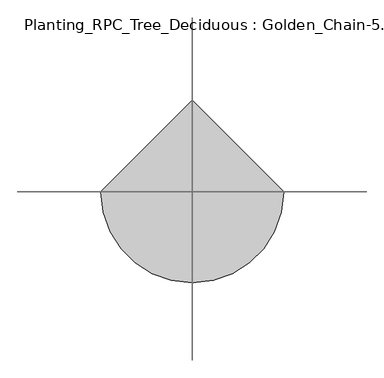
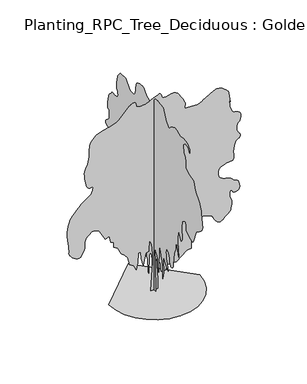
"""IFC4 building model written with IfcOpenShell, lengths in millimetres: geographic element geometry, Planting_RPC_Tree_Deciduous : Golden_Chain-5.5_Meters."""

from ifc_helpers import new_model, si_unit, origin, place, context, project, spatial, triangles, source, transform, mapped, element, save


def planting_rpc_tree_deciduous_golden_chain_5_5_meters_6778af60(model_context):
    return source(origin(), model_context, "Body", "Tessellation", [
        triangles([(-0.0021492, 84.2526153, 0.0017055), (-0.0021492, -79.7118042, 0.0017055), (-0.0021492, -55.1171299, 770.634066), (-0.0021492, -30.52271, 1205.1391577), (-0.0021492, -128.9011618, 1090.3648407), (-0.0021492, -161.6941456, 983.7870438), (-0.0021492, -161.6941456, 778.8331295), (-0.0021492, -202.6851937, 614.8669024), (-0.0021492, -227.2798771, 1410.0956154), (-0.0021492, -292.8648273, 1254.3285244), (-0.0021492, -391.2435245, 934.5977497), (-0.0021492, -407.6416878, 557.4810519), (-0.0021492, -448.6319547, 754.2384825), (-0.0021492, -424.0372713, 1123.1586239), (-0.0021492, -399.4426243, 1229.7338047), (-0.0021492, -563.4062716, 1024.7798904), (-0.0021492, -645.3893852, 910.00303), (-0.0021492, -571.6053351, 1164.1488544), (-0.0021492, -566.3701532, 1202.7023878), (-0.0021492, -561.3514189, 1240.6803749), (-0.0021492, -556.7629998, 1277.5125744), (-0.0021492, -552.8187638, 1312.6233673), (-0.0021492, -549.7351948, 1345.442585), (-0.0021492, -547.7261604, 1375.3895943), (-0.0021492, -547.0106518, 1401.8965519), (-0.0021492, -548.2048739, 1425.0576382), (-0.0021492, -551.550709, 1445.6369053), (-0.0021492, -556.6891308, 1464.0644142), (-0.0021492, -563.2636931, 1480.7706619), (-0.0021492, -570.9127539, 1496.1884708), (-0.0021492, -579.2773232, 1510.7457218), (-0.0021492, -588.000955, 1524.870005), (-0.0021492, -615.9185097, 1493.2475166), (-0.0021492, -642.6877333, 1461.6276443), (-0.0021492, -667.1627655, 1430.0051559), (-0.0021492, -688.1976734, 1398.3826675), (-0.0021492, -704.6416552, 1366.7627953), (-0.0021492, -715.3488504, 1335.1403069), (-0.0021492, -719.173399, 1303.5178185), (-0.0021492, -720.8463346, 1273.0922047), (-0.0021492, -725.5315138, 1244.8155876), (-0.0021492, -732.7248247, 1218.3340645), (-0.0021492, -741.9270973, 1193.2836313), (-0.0021492, -752.6342926, 1169.31024), (-0.0021492, -764.3472404, 1146.0549007), (-0.0021492, -776.5592857, 1123.1586239), (-0.0021492, -799.2416948, 1123.4208899), (-0.0021492, -820.9921841, 1125.2618385), (-0.0021492, -840.8787609, 1130.2576818), (-0.0021492, -857.9695055, 1139.9845591), (-0.0021492, -871.3298819, 1156.0210802), (-0.0021492, -880.0305862, 1179.9486168), (-0.0021492, -883.1370827, 1213.3382212), (-0.0021492, -884.8100183, 1255.5711811), (-0.0021492, -889.4951975, 1304.2589069), (-0.0021492, -896.6884357, 1358.3243568), (-0.0021492, -905.890781, 1416.6930325), (-0.0021492, -916.5979763, 1478.2854939), (-0.0021492, -928.3109241, 1542.0320389), (-0.0021492, -940.5255129, 1606.8530823), (-0.0021492, -1006.1104631, 1762.6177025), (-0.0021492, -1030.7051102, 2041.3581013), (-0.0021492, -1137.2829071, 1615.0495296), (-0.0021492, -1096.2900604, 2033.1590378), (-0.0021492, -1120.8847801, 2385.6835957), (-0.0021492, -1260.2563602, 2139.7368347), (-0.0021492, -1270.7241806, 2153.8611179), (-0.0021492, -1280.7616493, 2168.4183689), (-0.0021492, -1289.9410309, 2183.833707), (-0.0021492, -1297.8295029, 2200.5424255), (-0.0021492, -1303.9940975, 2218.9699345), (-0.0021492, -1308.0095501, 2239.5492016), (-0.0021492, -1309.4456543, 2262.7102879), (-0.0021492, -1307.6275967, 2290.0778034), (-0.0021492, -1302.9424175, 2322.033847), (-0.0021492, -1296.538448, 2357.1447853), (-0.0021492, -1289.5590775, 2393.9769848), (-0.0021492, -1283.1526371, 2431.0968121), (-0.0021492, -1278.467458, 2467.0683083), (-0.0021492, -1276.6518711, 2500.45784), (-0.0021492, -1277.8461296, 2532.7959824), (-0.0021492, -1281.1944717, 2566.4375336), (-0.0021492, -1286.3329662, 2601.1435547), (-0.0021492, -1292.9049488, 2636.6899315), (-0.0021492, -1300.5540459, 2672.8981865), (-0.0021492, -1308.9185062, 2709.5395546), (-0.0021492, -1317.642247, 2746.4096878), (-0.0021492, -1349.0965771, 2763.5973015), (-0.0021492, -1379.5477707, 2778.4931946), (-0.0021492, -1407.98993, 2788.7800667), (-0.0021492, -1433.4222439, 2792.1923584), (-0.0021492, -1454.8366344, 2786.4374771), (-0.0021492, -1471.2347614, 2769.1992851), (-0.0021492, -1481.6057854, 2738.2107697), (-0.0021492, -1484.4041611, 2701.900486), (-0.0021492, -1481.8935585, 2669.6135033), (-0.0021492, -1478.8100258, 2640.3309883), (-0.0021492, -1479.8871403, 2613.0602692), (-0.0021492, -1489.8532471, 2586.7825127), (-0.0021492, -1513.444685, 2560.5300453), (-0.0021492, -1555.3924152, 2533.2517685), (-0.0021492, -1606.8988644, 2505.0718025), (-0.0021492, -1655.253035, 2478.4681938), (-0.0021492, -1699.3015091, 2456.025087), (-0.0021492, -1737.903368, 2440.3219757), (-0.0021492, -1769.9076645, 2433.9411152), (-0.0021492, -1794.1662128, 2439.4615631), (-0.0021492, -1809.5357689, 2459.4676094), (-0.0021492, -1957.1037964, 2820.1761154), (-0.0021492, -2096.4727604, 2918.5648773), (-0.0021492, -2133.9033245, 2947.2108032), (-0.0021492, -2168.0337994, 2976.9770096), (-0.0021492, -2197.5760368, 3008.067263), (-0.0021492, -2221.2386913, 3040.5580124), (-0.0021492, -2237.731144, 3074.6530243), (-0.0021492, -2245.7620491, 3110.453746), (-0.0021492, -2244.0407879, 3148.1136566), (-0.0021492, -2235.2459759, 3194.9398682), (-0.0021492, -2223.869054, 3254.6760475), (-0.0021492, -2211.3438011, 3322.1530334), (-0.0021492, -2199.1063213, 3392.2013741), (-0.0021492, -2188.5901028, 3459.67836), (-0.0021492, -2181.2287788, 3519.4145393), (-0.0021492, -2178.4558376, 3566.2154617), (-0.0021492, -2170.3281361, 3608.6875786), (-0.0021492, -2147.5744377, 3658.060437), (-0.0021492, -2112.6315125, 3713.1367264), (-0.0021492, -2067.9338047, 3772.8217461), (-0.0021492, -2015.9257874, 3835.9446373), (-0.0021492, -1959.038998, 3901.3845383), (-0.0021492, -1899.7152935, 3967.9447197), (-0.0021492, -1842.3294067, 4197.4932083), (-0.0021492, -1629.1739582, 4246.6875893), (-0.0021492, -1457.0136818, 4328.652935), (-0.0021492, -1458.3505188, 4335.1970123), (-0.0021492, -1461.6963902, 4352.7409996), (-0.0021492, -1466.0480141, 4378.3565872), (-0.0021492, -1470.3970219, 4408.9631493), (-0.0021492, -1473.7428932, 4441.6065056), (-0.0021492, -1475.082201, 4473.2060303), (-0.0021492, -1473.409338, 4500.8334137), (-0.0021492, -1467.7438408, 4526.8565346), (-0.0021492, -1458.2079403, 4555.4515915), (-0.0021492, -1445.4433125, 4586.2107605), (-0.0021492, -1430.0993362, 4618.7015099), (-0.0021492, -1412.8176876, 4652.4654373), (-0.0021492, -1394.2474548, 4687.1205894), (-0.0021492, -1375.0306046, 4722.1829842), (-0.0021492, -1342.2368214, 4918.9352188), (-0.0021492, -1448.8146183, 5009.1250626), (-0.0021492, -1579.9871349, 4984.5277267), (-0.0021492, -1653.7685326, 4877.9400467), (-0.0021492, -1653.7685326, 4976.3288086), (-0.0021492, -1538.9942883, 5082.8914902), (-0.0021492, -1350.4358849, 5107.488826), (-0.0021492, -1202.8678574, 5074.692572), (-0.0021492, -1055.2998299, 5156.6829163), (-0.0021492, -948.7220329, 5164.8818344), (-0.0021492, -940.8819592, 5161.1390396), (-0.0021492, -920.1372952, 5151.1065125), (-0.0021492, -890.6409851, 5136.4911255), (-0.0021492, -856.5588358, 5118.9980072), (-0.0021492, -822.0437914, 5100.3334488), (-0.0021492, -791.2590425, 5082.280481), (-0.0021492, -768.3627657, 5066.4930725), (-0.0021492, -752.5400396, 5050.8591431), (-0.0021492, -739.1541561, 5033.7985565), (-0.0021492, -726.6289759, 5017.8844116), (-0.0021492, -713.3882143, 5005.6874817), (-0.0021492, -697.8532614, 4999.805864), (-0.0021492, -678.4453617, 5002.8359116), (-0.0021492, -653.5859053, 5017.2989822), (-0.0021492, -627.1527803, 5039.5790176), (-0.0021492, -603.7294281, 5064.0234558), (-0.0021492, -582.814135, 5090.2247635), (-0.0021492, -563.9078762, 5117.8777267), (-0.0021492, -546.5090472, 5146.6253906), (-0.0021492, -530.1108839, 5176.0602219), (-0.0021492, -514.2169049, 5205.8775879), (-0.0021492, -415.8382078, 5410.8290314), (-0.0021492, -169.8924643, 5451.8242035), (-0.0021492, -163.845268, 5451.6713058), (-0.0021492, -147.6161895, 5450.6783432), (-0.0021492, -124.0728773, 5447.9540909), (-0.0021492, -96.0842423, 5442.6323227), (-0.0021492, -66.5181736, 5433.8985535), (-0.0021492, -38.2425694, 5420.8359787), (-0.0021492, -14.1260625, 5402.6295319), (-0.0021492, 3.3458589, 5384.2457703), (-0.0021492, 15.2248406, 5370.0373352), (-0.0021492, 23.9488607, 5358.0950409), (-0.0021492, 31.9557643, 5346.6114395), (-0.0021492, 41.6836339, 5333.6761826), (-0.0021492, 55.5706269, 5317.4306625), (-0.0021492, 76.0543103, 5296.0418518), (-0.0021492, 97.13535, 5271.2916183), (-0.0021492, 113.1971331, 5247.5349289), (-0.0021492, 127.2514169, 5226.7827072), (-0.0021492, 142.3091915, 5211.0464584), (-0.0021492, 161.3827366, 5202.3638489), (-0.0021492, 187.483033, 5202.6946426), (-0.0021492, 223.6221062, 5214.076506), (-0.0021492, 264.351397, 5233.7851868), (-0.0021492, 302.4974698, 5257.3889786), (-0.0021492, 338.4919115, 5284.2012955), (-0.0021492, 372.7676173, 5313.5855484), (-0.0021492, 405.7523409, 5344.9307281), (-0.0021492, 437.8763975, 5377.549086), (-0.0021492, 469.5675954, 5410.8290314), (-0.0021492, 492.466452, 5419.4860611), (-0.0021492, 515.7217913, 5427.3286057), (-0.0021492, 539.6951463, 5433.618338), (-0.0021492, 564.7456158, 5437.5396103), (-0.0021492, 591.2271026, 5438.3035172), (-0.0021492, 619.503756, 5435.1205719), (-0.0021492, 649.9294424, 5427.2268677), (-0.0021492, 681.4067362, 5417.9076691), (-0.0021492, 712.0259428, 5409.8610672), (-0.0021492, 740.9213448, 5401.4075134), (-0.0021492, 767.2373257, 5390.7895569), (-0.0021492, 790.1107115, 5376.3009064), (-0.0021492, 808.6833424, 5356.2364334), (-0.0021492, 822.0921896, 5328.8381058), (-0.0021492, 831.6764156, 5297.4679276), (-0.0021492, 839.5393805, 5266.5047012), (-0.0021492, 845.9687845, 5235.9240097), (-0.0021492, 851.2523283, 5205.5973724), (-0.0021492, 855.672698, 5175.5253708), (-0.0021492, 859.522681, 5145.5556885), (-0.0021492, 863.0824202, 5115.6877441), (-0.0021492, 868.5086151, 5085.9976959), (-0.0021492, 874.8667299, 5057.4029297), (-0.0021492, 883.0886845, 5030.9469864), (-0.0021492, 894.1065439, 5007.6989868), (-0.0021492, 908.8546263, 4988.7803741), (-0.0021492, 928.2625259, 4975.2085281), (-0.0021492, 953.2646336, 4968.1298904), (-0.0021492, 983.5706326, 4964.7940475), (-0.0021492, 1017.0340696, 4962.6296448), (-0.0021492, 1051.7859455, 4962.7313828), (-0.0021492, 1085.9648186, 4966.2962814), (-0.0021492, 1117.7069944, 4974.4446213), (-0.0021492, 1145.1458719, 4988.347261), (-0.0021492, 1166.4176113, 5009.1250626), (-0.0021492, 1187.9516893, 5037.6180908), (-0.0021492, 1215.2250246, 5071.5857849), (-0.0021492, 1244.9327316, 5107.4120865), (-0.0021492, 1273.7822788, 5141.5326782), (-0.0021492, 1298.4736496, 5170.3309204), (-0.0021492, 1315.7070454, 5190.2430771), (-0.0021492, 1322.1822315, 5197.6786697), (-0.0021492, 1576.328056, 5181.2802521), (-0.0021492, 1674.7067894, 5058.2941544), (-0.0021492, 1679.9878624, 5049.3057495), (-0.0021492, 1685.3426228, 5039.1203247), (-0.0021492, 1690.840107, 5026.4652832), (-0.0021492, 1696.5540024, 5010.1691849), (-0.0021492, 1702.550584, 4988.9838501), (-0.0021492, 1708.9086262, 4961.7134216), (-0.0021492, 1715.69702, 4927.1347183), (-0.0021492, 1722.2461842, 4888.9655365), (-0.0021492, 1727.9344997, 4851.6622902), (-0.0021492, 1732.907452, 4815.0465019), (-0.0021492, 1737.304858, 4779.0417229), (-0.0021492, 1741.2720577, 4743.4444771), (-0.0021492, 1744.9539551, 4708.1530266), (-0.0021492, 1748.4908031, 4672.9886032), (-0.0021492, 1731.0893944, 4648.3403984), (-0.0021492, 1714.6937382, 4623.4122688), (-0.0021492, 1700.3046455, 4597.9237083), (-0.0021492, 1688.927869, 4571.5442139), (-0.0021492, 1681.5665451, 4544.0441483), (-0.0021492, 1679.2239555, 4515.0927177), (-0.0021492, 1682.9058529, 4484.4352867), (-0.0021492, 1691.9172215, 4457.546521), (-0.0021492, 1704.798848, 4438.9584114), (-0.0021492, 1721.4109154, 4426.9908279), (-0.0021492, 1741.6082291, 4419.8866104), (-0.0021492, 1765.2454491, 4415.940049), (-0.0021492, 1792.1827583, 4413.4445618), (-0.0021492, 1822.2748169, 4410.6435699), (-0.0021492, 1851.5776794, 4410.5162521), (-0.0021492, 1877.0099934, 4414.7177399), (-0.0021492, 1899.7152935, 4419.453788), (-0.0021492, 1920.8445271, 4421.0580505), (-0.0021492, 1941.543409, 4415.7871513), (-0.0021492, 1962.9576542, 4399.8982956), (-0.0021492, 1986.2385006, 4369.6483978), (-0.0021492, 2009.8529022, 4339.016256), (-0.0021492, 2031.6033188, 4320.2755394), (-0.0021492, 2051.6324741, 4307.2641243), (-0.0021492, 2070.0854176, 4293.8451759), (-0.0021492, 2087.1024021, 4273.8057014), (-0.0021492, 2102.8308025, 4241.0094475), (-0.0021492, 2117.4110172, 4189.2939995), (-0.0021492, 2130.4606567, 4132.1297562), (-0.0021492, 2141.5040234, 4085.4561516), (-0.0021492, 2150.5382103, 4046.6759605), (-0.0021492, 2157.565979, 4013.1922485), (-0.0021492, 2162.5848587, 3982.4330795), (-0.0021492, 2165.5945587, 3951.8009377), (-0.0021492, 2166.6003113, 3918.7500481), (-0.0021492, 2163.9699486, 3888.1437767), (-0.0021492, 2156.6086246, 3865.7361328), (-0.0021492, 2145.3030647, 3850.1274925), (-0.0021492, 2130.8426102, 3839.9676476), (-0.0021492, 2114.0167477, 3833.9075523), (-0.0021492, 2095.6120571, 3830.5464203), (-0.0021492, 2076.4181705, 3828.5602043), (-0.0021492, 2076.4181705, 3615.4098427), (-0.0021492, 2076.5861835, 3611.7687859), (-0.0021492, 2077.7574783, 3607.2362137), (-0.0021492, 2080.9351913, 3600.9979317), (-0.0021492, 2087.1278366, 3592.1877136), (-0.0021492, 2097.3334637, 3579.9143349), (-0.0021492, 2112.5576797, 3563.3636009), (-0.0021492, 2133.8065281, 3541.6437057), (-0.0021492, 2158.6890209, 3518.8288193), (-0.0021492, 2183.2835953, 3498.7640556), (-0.0021492, 2206.2996323, 3480.0997879), (-0.0021492, 2226.4484024, 3461.6134163), (-0.0021492, 2242.4391415, 3441.9561859), (-0.0021492, 2252.9807945, 3419.8796265), (-0.0021492, 2256.7799812, 3394.0602722), (-0.0021492, 2250.3276134, 3369.7687317), (-0.0021492, 2232.2566235, 3352.3773514), (-0.0021492, 2204.5070091, 3340.7152725), (-0.0021492, 2169.0142628, 3333.6366348), (-0.0021492, 2127.7106792, 3329.995578), (-0.0021492, 2082.5368378, 3328.6715309), (-0.0021492, 2035.4277946, 3328.4677643), (-0.0021492, 2021.5658501, 3329.995578), (-0.0021492, 2008.8496204, 3330.1737648), (-0.0021492, 1998.4275822, 3327.6274086), (-0.0021492, 1991.4508278, 3320.9815933), (-0.0021492, 1989.05984, 3308.886692), (-0.0021492, 1992.405566, 3289.9677887), (-0.0021492, 2002.6366276, 3262.9005455), (-0.0021492, 2020.3945553, 3234.9676575), (-0.0021492, 2044.3195484, 3213.2224731), (-0.0021492, 2072.5477673, 3195.7802238), (-0.0021492, 2103.212756, 3180.7570129), (-0.0021492, 2134.4508202, 3166.3195221), (-0.0021492, 2164.4003002, 3150.6088531), (-0.0021492, 2191.195031, 3131.7155296), (-0.0021492, 2214.6667088, 3115.4700096), (-0.0021492, 2235.4113728, 3106.0996513), (-0.0021492, 2252.7159851, 3099.4538361), (-0.0021492, 2265.8625664, 3091.381945), (-0.0021492, 2274.1329918, 3077.7083611), (-0.0021492, 2276.8091366, 3054.2824654), (-0.0021492, 2273.1754921, 3016.9539299), (-0.0021492, 2263.7593517, 2975.5765137), (-0.0021492, 2250.0398403, 2941.939904), (-0.0021492, 2232.735228, 2914.7709229), (-0.0021492, 2212.5634941, 2892.7455231), (-0.0021492, 2190.2375313, 2874.6158157), (-0.0021492, 2166.4806965, 2859.0580444), (-0.0021492, 2142.0055916, 2844.7731606), (-0.0021492, 2133.3761765, 2827.1783043), (-0.0021492, 2125.6812973, 2809.2779434), (-0.0021492, 2119.8477871, 2790.7918625), (-0.0021492, 2116.8125072, 2771.4654259), (-0.0021492, 2117.5051975, 2750.9675491), (-0.0021492, 2122.8599579, 2729.044178), (-0.0021492, 2133.8065281, 2705.4145157), (-0.0021492, 2153.6931049, 2682.9815826), (-0.0021492, 2182.4714355, 2663.4005104), (-0.0021492, 2215.980582, 2644.532476), (-0.0021492, 2250.062804, 2624.2386566), (-0.0021492, 2280.5623959, 2600.3543587), (-0.0021492, 2303.3160942, 2570.7407593), (-0.0021492, 2314.1683388, 2533.2517685), (-0.0021492, 2316.6306885, 2491.7827881), (-0.0021492, 2316.7960854, 2450.4562408), (-0.0021492, 2314.3822792, 2407.4085777), (-0.0021492, 2309.1012062, 2360.7782845), (-0.0021492, 2300.6627678, 2308.6964344), (-0.0021492, 2288.7842777, 2249.3015133), (-0.0021492, 2273.1754921, 2180.7272106), (-0.0021492, 2256.9479942, 2122.3126076), (-0.0021492, 2242.7269146, 2087.8459614), (-0.0021492, 2229.5091167, 2067.1470795), (-0.0021492, 2216.2913189, 2050.0334438), (-0.0021492, 2202.0702393, 2026.3248619), (-0.0021492, 2185.8401253, 1985.8335835), (-0.0021492, 2166.6003113, 1918.3847935), (-0.0021492, 2149.5808559, 1842.5203835), (-0.0021492, 2138.8736607, 1783.2936207), (-0.0021492, 2131.7517117, 1740.2713921), (-0.0021492, 2125.4903206, 1713.0234913), (-0.0021492, 2117.362619, 1701.1195667), (-0.0021492, 2104.6463894, 1704.1317375), (-0.0021492, 2084.617234, 1721.6273266), (-0.0021492, 2060.5012642, 1758.0775726), (-0.0021492, 2037.2458523, 1813.4570412), (-0.0021492, 2014.7060944, 1880.5977104), (-0.0021492, 1992.7391212, 1952.324437), (-0.0021492, 1971.2051159, 2021.4716698), (-0.0021492, 1949.9562675, 2080.8664455), (-0.0021492, 1928.8526138, 2123.3387077), (-0.0021492, 1903.2291779, 2154.4824463), (-0.0021492, 1869.4322582, 2184.7680977), (-0.0021492, 1828.8238358, 2214.3331535), (-0.0021492, 1782.7664726, 2243.3252792), (-0.0021492, 1732.6196789, 2271.8870533), (-0.0021492, 1679.7509583, 2300.1636703), (-0.0021492, 1625.51735, 2328.2952381), (-0.0021492, 1580.1042789, 2357.6693172), (-0.0021492, 1536.2697453, 2384.1049129), (-0.0021492, 1495.5901062, 2404.6612164), (-0.0021492, 1459.6414284, 2416.3971279), (-0.0021492, 1430.0025398, 2416.3715481), (-0.0021492, 1408.2521233, 2401.6489002), (-0.0021492, 1395.9662453, 2369.2854687), (-0.0021492, 1387.7442181, 2327.3633183), (-0.0021492, 1377.3731941, 2285.8713741), (-0.0021492, 1365.2069309, 2244.7359489), (-0.0021492, 1351.6071796, 2203.8882969), (-0.0021492, 1336.9303139, 2163.2544399), (-0.0021492, 1321.5379395, 2122.7657776), (-0.0021492, 1305.7865753, 2082.3484772), (-0.0021492, 1125.4248373, 1926.583857), (-0.0021492, 1107.9775738, 1907.1276318), (-0.0021492, 1091.2458916, 1886.8820652), (-0.0021492, 1075.9502409, 1865.0602867), (-0.0021492, 1062.8037323, 1840.8729549), (-0.0021492, 1052.5268887, 1813.5282578), (-0.0021492, 1045.8352186, 1782.2419407), (-0.0021492, 1043.4442308, 1746.2220463), (-0.0021492, 1042.7261787, 1711.1595062), (-0.0021492, 1040.7196878, 1682.5468632), (-0.0021492, 1037.6361551, 1659.3168858), (-0.0021492, 1033.6919191, 1640.3851925), (-0.0021492, 1029.1035364, 1624.6822266), (-0.0021492, 1024.0847294, 1611.1308735), (-0.0021492, 1018.8495838, 1598.6540188), (-0.0021492, 871.2814837, 1500.2752853), (-0.0021492, 854.8859001, 1328.1125381), (-0.0021492, 731.9125196, 1270.7241806), (-0.0021492, 699.1188091, 1057.5711302), (-0.0021492, 567.9463288, 1024.7798904), (-0.0021492, 579.9928319, 1019.3537682), (-0.0021492, 590.5345213, 1012.9956533), (-0.0021492, 598.0638946, 1004.7736261), (-0.0021492, 601.0736309, 993.7558393), (-0.0021492, 598.0638946, 979.0076843), (-0.0021492, 587.5222415, 959.5997847), (-0.0021492, 567.9463288, 934.5977497), (-0.0021492, 544.3090362, 908.8801334), (-0.0021492, 522.3905339, 887.4631994), (-0.0021492, 501.9081359, 869.6340551), (-0.0021492, 482.5715618, 854.6720324), (-0.0021492, 464.0956183, 841.8616224), (-0.0021492, 446.192605, 830.4822298), (-0.0021492, 428.5773285, 819.8234327), (-0.0021492, 416.3169213, 852.4974558), (-0.0021492, 404.2703819, 880.9396151), (-0.0021492, 392.6541942, 900.9203722), (-0.0021492, 381.6821895, 908.2104795), (-0.0021492, 371.5733952, 898.5777826), (-0.0021492, 362.5365921, 867.7931065), (-0.0021492, 354.7933147, 811.6243692), (-0.0021492, 347.289376, 757.5588467), (-0.0021492, 338.9222268, 728.4470335), (-0.0021492, 329.8396053, 713.1030573), (-0.0021492, 320.1840537, 700.3409729), (-0.0021492, 310.0981504, 678.9725098), (-0.0021492, 299.7245467, 637.8141209), (-0.0021492, 289.2083463, 565.677572), (-0.0021492, 280.1002358, 485.3215393), (-0.0021492, 273.5766333, 424.7553234), (-0.0021492, 269.2021002, 380.6814875), (-0.0021492, 266.5488464, 349.8000149), (-0.0021492, 265.1865749, 328.815976), (-0.0021492, 264.6849704, 314.426847), (-0.0021492, 264.613663, 303.3351912), (-0.0021492, 240.0187434, 811.6243692), (-0.0021492, 227.6618124, 844.6574547), (-0.0021492, 214.9461096, 875.6102165), (-0.0021492, 201.5133903, 902.4023312), (-0.0021492, 187.005355, 922.9585619), (-0.0021492, 171.062996, 935.1961143), (-0.0021492, 153.328032, 937.037063), (-0.0021492, 133.4419729, 926.401157), (-0.0021492, 115.707018, 904.291678), (-0.0021492, 103.9950694, 874.0085701), (-0.0021492, 97.3026454, 836.9141773), (-0.0021492, 94.6257194, 794.3680824), (-0.0021492, 94.9603011, 747.7377892), (-0.0021492, 97.3026454, 698.3803368), (-0.0021492, 100.6487348, 647.6606855), (-0.0021492, 84.2526153, 237.7499866), (88.4435659, 0.0002505, 0.0), (-86.3932913, 0.0002505, 0.0), (-44.7656723, 0.0002025, 807.5807934), (-36.4400473, 0.0001919, 1032.3704155), (-69.7422955, 0.0001759, 1307.1158546), (-128.0216733, 0.0001652, 1448.6490761), (-144.6726646, 0.0001865, 1140.6032713), (-227.9278935, 0.0001865, 1115.6266708), (-294.532658, 0.0002025, 799.2544121), (-352.8122947, 0.0001919, 999.0699772), (-361.138676, 0.0001812, 1182.2301636), (-427.7421324, 0.0001812, 1182.2301636), (-444.3923879, 0.0001972, 915.8137218), (-486.0217873, 0.0002079, 732.6509193), (-552.6252437, 0.0002025, 874.1842861), (-660.8581358, 0.0001972, 940.7903223), (-702.4849554, 0.0001812, 1157.2534904), (-785.7412107, 0.0001759, 1257.1625084), (-877.3238474, 0.0001759, 1332.0923824), (-977.2303219, 0.0001599, 1523.5789501), (-1085.4632504, 0.0001599, 1581.8586777), (-1085.4632504, 0.0001492, 1723.3945152), (-1160.3931244, 0.0001492, 1748.3711884), (-1202.019944, 0.0001386, 1939.857756), (-1318.5792538, 0.0001386, 1889.9044098), (-1468.4390018, 0.0001226, 2172.9736141), (-1502.3250149, 0.0001226, 2194.0442757), (-1536.1347244, 0.0001226, 2213.0727654), (-1569.8018555, 0.0001173, 2228.0246143), (-1603.2501045, 0.0001173, 2236.8602669), (-1636.4053482, 0.0001173, 2237.5401672), (-1669.1991314, 0.0001173, 2228.0246143), (-1701.5548599, 0.0001226, 2206.2766685), (-1733.4726791, 0.0001226, 2179.018594), (-1764.2269066, 0.0001226, 2153.3621658), (-1792.651189, 0.0001279, 2127.850787), (-1817.579464, 0.0001279, 2101.0306217), (-1837.8479942, 0.0001279, 2071.4426022), (-1852.2879559, 0.0001332, 2037.6304218), (-1859.7409893, 0.0001332, 1998.1373383), (-1862.0709343, 0.0001386, 1954.9318359), (-1863.0894768, 0.0001386, 1911.4359444), (-1864.5459286, 0.0001439, 1868.3754913), (-1868.1871307, 0.0001439, 1826.4812462), (-1875.759779, 0.0001439, 1786.4790367), (-1889.0133305, 0.0001492, 1749.0993416), (-1909.6943356, 0.0001492, 1715.0681339), (-1930.6655846, 0.0001546, 1683.7079842), (-1945.9586918, 0.0001546, 1654.8226833), (-1959.0644325, 0.0001546, 1629.87159), (-1973.4840466, 0.0001546, 1610.3057785), (-1992.7085999, 0.0001599, 1597.5870781), (-2020.2341, 0.0001599, 1593.1693245), (-2059.5539383, 0.0001599, 1598.5088242), (-2106.0849644, 0.0001546, 1614.4818317), (-2151.4523987, 0.0001546, 1639.6289886), (-2193.4662586, 0.0001546, 1671.9108845), (-2229.9496422, 0.0001492, 1709.2905796), (-2258.7125668, 0.0001492, 1749.7308437), (-2277.5730434, 0.0001439, 1791.1870342), (-2284.3435604, 0.0001439, 1831.6274437), (-2284.0049183, 0.0001439, 1867.2347179), (-2283.6662762, 0.0001386, 1899.34613), (-2284.3435604, 0.0001386, 1933.6447632), (-2287.0630165, 0.0001332, 1975.8062885), (-2292.8405708, 0.0001332, 2031.5116093), (-2302.6947659, 0.0001279, 2106.4440994), (-2317.6466148, 0.0001226, 2206.2766685), (-2328.3767738, 0.0001119, 2318.4664776), (-2327.0169731, 0.0001066, 2424.8304794), (-2316.773267, 0.0001013, 2522.6006744), (-2300.8512737, 9.59e-05, 2609.0116791), (-2282.4516701, 9.06e-05, 2681.301162), (-2264.780365, 9.06e-05, 2736.6829559), (-2251.0431221, 8.53e-05, 2772.4075195), (-2228.7604706, 8.53e-05, 2807.0370918), (-2187.9815643, 7.99e-05, 2856.639006), (-2135.6984184, 7.99e-05, 2914.8473717), (-2078.9007225, 7.46e-05, 2975.2454292), (-2024.5780209, 7.46e-05, 3031.4167099), (-1979.7200031, 6.93e-05, 3076.9444542), (-1951.3211552, 6.93e-05, 3105.4374825), (-1924.2819626, 6.4e-05, 3127.0812195), (-1882.823156, 6.4e-05, 3155.2940323), (-1832.9183533, 6.4e-05, 3188.4469505), (-1780.5385563, 5.86e-05, 3224.9607101), (-1731.6521507, 5.86e-05, 3263.2060501), (-1692.2328999, 5.33e-05, 3301.6042877), (-1668.2519508, 5.33e-05, 3338.5511604), (-1656.1646072, 5.33e-05, 3371.3218346), (-1648.0088551, 4.8e-05, 3398.84748), (-1643.1300831, 4.8e-05, 3421.9931602), (-1640.8716454, 4.8e-05, 3441.6759705), (-1640.5812561, 4.8e-05, 3458.7106865), (-1641.5997986, 4.8e-05, 3473.988533), (-1643.2752777, 4.26e-05, 3488.4260239), (-1673.4947994, 4.26e-05, 3483.4862091), (-1703.0597099, 4.26e-05, 3481.1180397), (-1731.3135086, 4.26e-05, 3483.8172935), (-1757.6014389, 4.26e-05, 3494.1806145), (-1781.2667095, 4.26e-05, 3514.7546494), (-1801.6574707, 4.26e-05, 3548.0601746), (-1818.1141697, 3.73e-05, 3596.6435463), (-1832.6281094, 3.2e-05, 3658.2386238), (-1846.5614159, 3.2e-05, 3726.3519081), (-1858.3075012, 2.66e-05, 3797.4190819), (-1866.2698059, 2.13e-05, 3867.7223488), (-1868.8440674, 1.6e-05, 3933.671521), (-1864.4261684, 1.6e-05, 3991.625251), (-1851.414608, 1.07e-05, 4037.8913223), (-1831.8514126, 1.07e-05, 4080.6180748), (-1810.1034668, 5.3e-06, 4129.8889046), (-1788.0628063, 5.3e-06, 4185.1436714), (-1767.626263, 0.0, 4245.7710754), (-1750.6831112, -5.3e-06, 4311.2106857), (-1739.1280025, -1.07e-05, 4380.8773636), (-1734.8579144, -1.07e-05, 4454.1853889), (-1735.4894165, -1.6e-05, 4523.877356), (-1735.8280586, -2.13e-05, 4584.5303398), (-1733.5466572, -2.13e-05, 4638.3334511), (-1726.3125057, -2.66e-05, 4687.5025429), (-1711.7987114, -3.2e-05, 4734.1761475), (-1687.6699516, -3.2e-05, 4780.5442474), (-1651.601659, -3.73e-05, 4828.8218239), (-1604.6581581, -3.73e-05, 4875.2407928), (-1551.3056007, -4.26e-05, 4914.6575729), (-1494.3144573, -4.26e-05, 4947.2247711), (-1436.4472046, -4.26e-05, 4973.1202835), (-1380.4746037, -4.26e-05, 4992.421431), (-1329.161602, -4.8e-05, 5005.3566879), (-1285.2761993, -4.8e-05, 5012.0022125), (-1238.819006, -4.8e-05, 5019.8197586), (-1181.7285227, -4.8e-05, 5034.7665207), (-1119.6854347, -4.8e-05, 5054.8059952), (-1058.3731888, -4.8e-05, 5077.9260956), (-1003.4673832, -5.33e-05, 5102.03974), (-960.651392, -5.33e-05, 5125.1598404), (-935.6009588, -5.33e-05, 5145.1993149), (-669.1845171, -6.93e-05, 5428.27099), (-646.0030106, -6.93e-05, 5444.1601364), (-622.8954094, -7.46e-05, 5458.928421), (-599.9328938, -7.46e-05, 5471.5328842), (-577.1893693, -7.46e-05, 5480.8520828), (-554.7386684, -7.46e-05, 5485.7918976), (-532.6495734, -7.46e-05, 5485.2826263), (-510.9983877, -7.46e-05, 5478.2295685), (-495.8275477, -7.46e-05, 5462.4933197), (-489.5407585, -6.93e-05, 5439.0418442), (-486.7500132, -6.93e-05, 5411.3888809), (-482.064834, -6.93e-05, 5382.9725922), (-470.0972506, -6.93e-05, 5357.3567139), (-445.4618357, -6.4e-05, 5337.9794083), (-402.7655319, -6.4e-05, 5328.3544144), (-352.1553217, -6.4e-05, 5326.9794983), (-306.7905035, -6.4e-05, 5329.5258545), (-265.7951497, -6.4e-05, 5335.3568939), (-228.2925333, -6.4e-05, 5343.8104477), (-193.4123404, -6.4e-05, 5354.2249283), (-160.2801876, -6.93e-05, 5365.9375854), (-128.0216733, -6.93e-05, 5378.3124115), (-76.4902348, -6.93e-05, 5408.3588333), (-26.1968067, -6.93e-05, 5436.7501236), (21.6206779, -7.46e-05, 5461.7805725), (65.7244948, -7.46e-05, 5481.7688873), (104.8766017, -7.46e-05, 5495.0605179), (137.8389157, -7.46e-05, 5500.0003326), (163.3739486, -7.46e-05, 5494.8820404), (179.7578323, -7.46e-05, 5482.2525787), (188.4231282, -7.46e-05, 5466.2872742), (192.8648993, -7.46e-05, 5447.6994553), (196.5786624, -6.93e-05, 5427.2012878), (203.0594986, -6.93e-05, 5405.5578415), (215.8026888, -6.93e-05, 5383.4562836), (238.3035501, -6.93e-05, 5361.6599396), (275.7078804, -6.4e-05, 5352.0093658), (327.5301169, -6.93e-05, 5359.8263306), (388.8194718, -6.93e-05, 5376.0974304), (454.6234131, -6.93e-05, 5391.7569397), (519.9893723, -6.93e-05, 5397.8426147), (579.9673974, -6.93e-05, 5385.2643127), (629.6048836, -6.4e-05, 5345.0068863), (669.510442, -6.4e-05, 5289.625383), (704.1731518, -5.86e-05, 5237.2989258), (734.4638901, -5.86e-05, 5187.5188248), (761.2611643, -5.33e-05, 5139.7758087), (785.4382496, -5.33e-05, 5093.5606064), (807.8660231, -4.8e-05, 5048.3633652), (829.420376, -4.8e-05, 5003.6759766), (821.0939947, -3.73e-05, 4853.8011131), (1104.163199, -3.73e-05, 4837.1483505), (1130.912075, -3.73e-05, 4839.0834068), (1157.5870457, -3.73e-05, 4841.7826607), (1184.116967, -3.73e-05, 4846.1111755), (1210.4303318, -3.73e-05, 4852.8334396), (1236.4509819, -3.73e-05, 4862.7639381), (1262.10741, -3.73e-05, 4876.6921577), (1287.3259289, -3.73e-05, 4895.433165), (1317.642247, -4.26e-05, 4918.5532654), (1357.5732399, -4.26e-05, 4944.7039948), (1405.5097034, -4.26e-05, 4973.4260788), (1459.8579849, -4.8e-05, 5004.1852478), (1519.010915, -4.8e-05, 5036.4722305), (1581.3671379, -4.8e-05, 5069.7527573), (1645.3250072, -5.33e-05, 5103.5675537), (1684.4540142, -5.33e-05, 5099.8497574), (1722.8521065, -5.33e-05, 5095.2663162), (1759.7963631, -5.33e-05, 5088.9515854), (1794.5558693, -4.8e-05, 5079.9887604), (1826.3998558, -4.8e-05, 5067.5371948), (1854.6051109, -4.8e-05, 5050.7062454), (1878.4410107, -4.8e-05, 5028.6552658), (1900.2143909, -4.8e-05, 5007.1897156), (1922.1329659, -4.26e-05, 4990.5372437), (1943.3232422, -4.26e-05, 4975.3358459), (1962.9118721, -4.26e-05, 4958.2502609), (1980.023037, -4.26e-05, 4935.9190659), (1993.7857143, -3.73e-05, 4905.0069992), (2003.3267017, -3.73e-05, 4862.1273491), (2036.62714, -2.13e-05, 4620.6877258), (2031.3358932, -2.66e-05, 4643.2223969), (2026.4088684, -2.66e-05, 4661.7340576), (2022.2099968, -2.66e-05, 4672.2502762), (2019.1035004, -2.66e-05, 4670.7477516), (2017.450985, -2.66e-05, 4653.2293442), (2017.6216141, -2.13e-05, 4615.6714622), (2019.9769936, -2.13e-05, 4554.0766754), (2029.0544918, -1.6e-05, 4483.8242775), (2046.7257969, -1.07e-05, 4423.1715843), (2069.3470905, -5.3e-06, 4372.5511276), (2093.2796413, -5.3e-06, 4332.4213097), (2114.8825378, -5.3e-06, 4303.2408234), (2130.5141418, -5.3e-06, 4285.3913315), (2136.5336872, 0.0, 4279.3565254), (2147.5539448, 0.0, 4280.1460121), (2175.7593452, 0.0, 4279.6367409), (2213.8671936, 0.0, 4273.4493279), (2254.5977016, 0.0, 4257.2038078), (2290.6659943, 0.0, 4226.5463768), (2314.794754, 5.3e-06, 4177.0973602), (2319.6963444, 1.07e-05, 4104.5023727), (2308.0216209, 1.07e-05, 4035.0650414), (2289.5024025, 1.6e-05, 3991.3959045), (2267.4871765, 1.6e-05, 3963.6159142), (2245.3241398, 1.6e-05, 3941.7939903), (2226.3694828, 2.13e-05, 3916.0255051), (2213.96399, 2.13e-05, 3876.4308289), (2211.466032, 2.66e-05, 3813.104171), (2219.5963497, 2.66e-05, 3747.2826073), (2234.7188278, 3.2e-05, 3702.4167412), (2253.6250866, 3.2e-05, 3671.9886566), (2273.1169201, 3.73e-05, 3649.4284058), (2289.9862392, 3.73e-05, 3628.141333), (2301.0320766, 3.73e-05, 3601.6598099), (2303.0461979, 4.26e-05, 3563.3380211), (2294.2843781, 4.26e-05, 3529.0395332), (2276.7837021, 4.26e-05, 3512.233873), (2253.0190189, 4.26e-05, 3502.8382256), (2225.4707005, 4.26e-05, 3490.8194824), (2196.6083633, 4.8e-05, 3466.1204086), (2168.9148502, 4.8e-05, 3418.7340569), (2144.8600685, 5.33e-05, 3338.5511604), (2129.882785, 5.86e-05, 3243.8796135), (2124.958231, 6.4e-05, 3160.284716), (2125.8545425, 6.93e-05, 3088.6321129), (2128.3549713, 7.46e-05, 3029.812738), (2128.2327404, 7.46e-05, 2984.6666565), (2121.2660145, 7.46e-05, 2954.0856743), (2103.2331036, 7.99e-05, 2938.9351456), (2080.3674934, 7.99e-05, 2933.5625084), (2059.979203, 7.99e-05, 2930.6853584), (2039.4433926, 7.99e-05, 2928.6482735), (2016.1421986, 7.99e-05, 2925.9237305), (1987.4504906, 7.99e-05, 2920.8565979), (1950.7506958, 7.99e-05, 2911.8426132), (1903.4176838, 7.99e-05, 2897.3033844), (1853.5127357, 7.99e-05, 2880.1413506), (1811.035532, 7.99e-05, 2862.9793167), (1776.2784966, 8.53e-05, 2843.7801979), (1749.5296932, 8.53e-05, 2820.5069092), (1731.0818367, 8.53e-05, 2791.0973671), (1721.2276417, 9.06e-05, 2753.5647743), (1720.2574974, 9.06e-05, 2705.8217583), (1723.631274, 9.59e-05, 2658.5115646), (1727.8785439, 9.59e-05, 2621.9722252), (1734.8910519, 9.59e-05, 2593.7338326), (1746.5683914, 0.0001013, 2571.3520592), (1764.7947498, 0.0001013, 2552.2802582), (1791.4723366, 0.0001013, 2534.1046234), (1828.4878098, 0.0001013, 2514.3224007), (1873.0047146, 0.0001013, 2496.0453186), (1919.5611752, 0.0001066, 2482.2824959), (1966.1151649, 0.0001066, 2470.414325), (2010.6320698, 0.0001066, 2457.815094), (2051.0697178, 0.0001066, 2441.8678116), (2085.3913147, 0.0001066, 2419.9517075), (2111.5570141, 0.0001119, 2389.4394711), (2135.660194, 0.0001119, 2361.79174), (2163.6949654, 0.0001119, 2345.6507195), (2193.4790485, 0.0001119, 2334.1695889), (2222.8250771, 0.0001119, 2320.5060333), (2249.5484459, 0.0001173, 2297.8084362), (2271.4670208, 0.0001173, 2259.2397148), (2286.3959061, 0.0001226, 2197.9502872), (2290.3019176, 0.0001279, 2132.9738754), (2281.9781525, 0.0001279, 2085.9081436), (2263.4563179, 0.0001279, 2053.7712971), (2236.7813473, 0.0001332, 2033.5767448), (2203.9875641, 0.0001332, 2022.3373146), (2167.1171402, 0.0001332, 2017.0716476), (2128.2097767, 0.0001332, 2014.7876301), (2106.9227039, 0.0001332, 2046.2216125), (2086.3639297, 0.0001279, 2073.5764835), (2067.2591366, 0.0001279, 2092.7780731), (2050.3415646, 0.0001279, 2099.7421829), (2036.3368961, 0.0001279, 2090.3972591), (2025.9709591, 0.0001279, 2060.6641903), (2019.9769936, 0.0001332, 2006.4637196), (2022.3322277, 0.0001386, 1947.8937481), (2033.7142365, 0.0001386, 1903.8861145), (2049.9035099, 0.0001439, 1868.6174824), (2066.6760326, 0.0001439, 1836.2616085), (2079.809824, 0.0001439, 1800.992831), (2085.075491, 0.0001492, 1756.9878136), (2078.2539597, 0.0001492, 1698.4178421), (2066.069965, 0.0001546, 1638.7046265), (2056.21577, 0.0001599, 1592.8306824), (2045.9236656, 0.0001599, 1557.2944794), (2032.4282684, 0.0001599, 1528.6053875), (2012.9618694, 0.0001652, 1503.2646378), (1984.7566143, 0.0001652, 1477.7762226), (1945.0471195, 0.0001652, 1448.6490761), (1902.3507431, 0.0001705, 1414.6917011), (1865.4803192, 0.0001705, 1379.8609783), (1832.1060482, 0.0001705, 1348.3784523), (1799.895369, 0.0001759, 1324.4688652), (1766.5210979, 0.0001759, 1312.3585579), (1729.6508194, 0.0001759, 1316.2645695), (1686.954443, 0.0001705, 1340.416293), (1647.1227173, 0.0001705, 1378.2109337), (1618.0669327, 0.0001705, 1418.4780979), (1596.2935524, 0.0001652, 1458.6025383), (1578.3090397, 0.0001652, 1495.9567989), (1560.6149162, 0.0001599, 1527.9254871), (1539.7148838, 0.0001599, 1551.8810017), (1512.115551, 0.0001599, 1565.2083858), (1471.7517357, 0.0001599, 1577.5375751), (1418.5696621, 0.0001599, 1596.5685356), (1358.1053295, 0.0001546, 1616.7632332), (1295.8943012, 0.0001546, 1632.58843), (1237.4695244, 0.0001546, 1638.511179), (1188.3667076, 0.0001546, 1628.9956261), (1154.1164726, 0.0001599, 1598.5088242), (1127.3931038, 0.0001599, 1577.4407787), (1098.3373192, 0.0001599, 1588.9958874), (1068.7009741, 0.0001546, 1616.8600296), (1040.2282934, 0.0001546, 1644.7266426), (1014.6711325, 0.0001546, 1656.2792805), (993.7711, 0.0001546, 1635.211235), (979.2801241, 0.0001599, 1565.2083858), (971.8780323, 0.0001652, 1477.5598114), (970.009033, 0.0001705, 1410.4444313), (972.0715525, 0.0001705, 1357.8940052), (976.4639442, 0.0001759, 1313.9347698), (981.5871054, 0.0001759, 1272.5981941), (985.8343025, 0.0001812, 1227.9132763), (987.6065054, 0.0001812, 1173.9063257), (995.9303432, 0.0002025, 832.5574665), (871.0472683, 0.0002025, 807.5807934), (729.5139015, 0.0002132, 691.0215563), (587.9780276, 0.0002185, 591.1150818), (396.4889165, 0.0002185, 599.4414631), (329.8854238, 0.0002185, 557.8146071), (304.9088233, 0.0002238, 457.9055892), (278.3305583, 0.0002238, 452.8104424), (252.8434148, 0.0002238, 449.2405294), (229.5414941, 0.0002238, 448.7312582), (209.5163901, 0.0002238, 452.8104424), (193.8604962, 0.0002238, 463.0032432), (183.6658786, 0.0002238, 480.845141), (180.0249308, 0.0002238, 507.8588264), (179.9037354, 0.0002185, 542.6437672), (179.0540417, 0.0002185, 581.2125249), (176.7483685, 0.0002132, 621.2377344), (172.257963, 0.0002132, 660.3896324), (164.854872, 0.0002132, 696.3382376), (153.8105607, 0.0002079, 726.7512068), (138.3973209, 0.0002079, 749.3012112), (121.7702562, 0.0002079, 768.113217), (107.3279238, 0.0002079, 788.6719912), (94.7059289, 0.0002025, 810.6872898), (83.5404222, 0.0002025, 833.8687963), (73.4672725, 0.0002025, 857.9236507), (64.1223624, 0.0002025, 882.5590656), (55.1413199, 0.0001972, 907.4872679), (63.4669473, 0.0002132, 691.0215563), (88.4435659, 0.0002345, 266.4189852), (-1216.0703945, 0.0, 0.0051165), (-1183.9209034, -278.6437659, 0.0051165), (-1092.3611578, -534.5312536, 0.0051165), (-948.7220329, -760.3342587, 0.0051165), (-760.3342587, -948.7220329, 0.0051165), (-534.5312536, -1092.3611578, 0.0051165), (-278.6437659, -1183.9209034, 0.0051165), (5.32e-05, -1216.0703945, 0.0051165), (278.6437659, -1183.9209034, 0.0051165), (534.5312536, -1092.3611578, 0.0051165), (760.3342587, -948.7220329, 0.0051165), (948.7220329, -760.3342587, 0.0051165), (1092.3611578, -534.5312536, 0.0051165), (1183.9209034, -278.6437659, 0.0051165), (1216.0703945, 0.0001066, 0.0051165), (-0.0001595, 1216.0703945, 0.0051165)], [[476, 477, 478], [475, 476, 478], [474, 475, 478], [473, 474, 478], [62, 63, 64], [472, 473, 478], [471, 472, 478], [470, 471, 478], [11, 12, 13], [11, 13, 14], [7, 8, 9], [6, 7, 9], [16, 17, 18], [469, 470, 478], [5, 6, 9], [10, 11, 14], [10, 14, 15], [468, 469, 478], [151, 152, 153], [151, 153, 154], [15, 16, 18], [467, 468, 478], [150, 151, 154], [150, 154, 155], [4, 5, 9], [15, 18, 19], [65, 66, 67], [65, 67, 68], [65, 68, 69], [65, 69, 70], [65, 70, 71], [65, 71, 72], [65, 72, 73], [65, 73, 74], [65, 74, 75], [65, 75, 76], [65, 76, 77], [466, 467, 478], [465, 466, 478], [464, 465, 478], [463, 464, 478], [15, 19, 20], [455, 456, 457], [65, 77, 78], [149, 150, 155], [149, 155, 156], [15, 20, 21], [62, 64, 65], [1, 2, 3], [493, 1, 3], [492, 493, 3], [491, 492, 3], [490, 491, 3], [489, 490, 3], [489, 3, 4], [488, 489, 4], [487, 488, 4], [486, 487, 4], [485, 486, 4], [484, 485, 4], [462, 463, 478], [462, 478, 479], [65, 78, 79], [15, 21, 22], [462, 479, 480], [461, 462, 480], [461, 480, 481], [391, 392, 393], [454, 455, 457], [440, 441, 442], [15, 22, 23], [65, 79, 80], [391, 393, 394], [390, 391, 394], [390, 394, 395], [389, 390, 395], [389, 395, 396], [388, 389, 396], [388, 396, 397], [387, 388, 397], [387, 397, 398], [386, 387, 398], [386, 398, 399], [385, 386, 399], [385, 399, 400], [384, 385, 400], [131, 132, 133], [45, 46, 47], [438, 439, 440], [383, 384, 400], [383, 400, 401], [382, 383, 401], [381, 382, 401], [380, 381, 401], [379, 380, 401], [379, 401, 402], [378, 379, 402], [378, 402, 403], [377, 378, 403], [376, 377, 403], [376, 403, 404], [375, 376, 404], [374, 375, 404], [373, 374, 404], [372, 373, 404], [371, 372, 404], [370, 371, 404], [369, 370, 404], [368, 369, 404], [367, 368, 404], [367, 404, 405], [366, 367, 405], [366, 405, 406], [366, 406, 407], [365, 366, 407], [365, 407, 408], [365, 408, 409], [364, 365, 409], [364, 409, 410], [363, 364, 410], [363, 410, 411], [15, 23, 24], [10, 15, 24], [9, 10, 24], [9, 24, 25], [9, 25, 26], [9, 26, 27], [9, 27, 28], [9, 28, 29], [179, 180, 181], [454, 457, 458], [453, 454, 458], [452, 453, 458], [461, 481, 482], [452, 458, 459], [451, 452, 459], [250, 251, 252], [9, 29, 30], [65, 80, 81], [460, 461, 482], [249, 250, 252], [249, 252, 253], [248, 249, 253], [247, 248, 253], [246, 247, 253], [246, 253, 254], [246, 254, 255], [246, 255, 256], [246, 256, 257], [246, 257, 258], [246, 258, 259], [246, 259, 260], [245, 246, 260], [245, 260, 261], [244, 245, 261], [244, 261, 262], [244, 262, 263], [244, 263, 264], [243, 244, 264], [243, 264, 265], [243, 265, 266], [243, 266, 267], [243, 267, 268], [243, 268, 269], [243, 269, 270], [243, 270, 271], [243, 271, 272], [242, 243, 272], [242, 272, 273], [241, 242, 273], [362, 363, 411], [450, 451, 459], [362, 411, 412], [483, 484, 4], [9, 30, 31], [241, 273, 274], [240, 241, 274], [449, 450, 459], [449, 459, 460], [448, 449, 460], [447, 448, 460], [446, 447, 460], [445, 446, 460], [444, 445, 460], [443, 444, 460], [442, 443, 460], [361, 362, 412], [9, 31, 32], [65, 81, 82], [106, 107, 108], [105, 106, 108], [105, 108, 109], [104, 105, 109], [103, 104, 109], [102, 103, 109], [101, 102, 109], [100, 101, 109], [99, 100, 109], [98, 99, 109], [97, 98, 109], [96, 97, 109], [95, 96, 109], [94, 95, 109], [93, 94, 109], [92, 93, 109], [45, 47, 48], [44, 45, 48], [44, 48, 49], [44, 49, 50], [44, 50, 51], [44, 51, 52], [44, 52, 53], [43, 44, 53], [43, 53, 54], [42, 43, 54], [41, 42, 54], [40, 41, 54], [40, 54, 55], [39, 40, 55], [38, 39, 55], [38, 55, 56], [37, 38, 56], [37, 56, 57], [36, 37, 57], [36, 57, 58], [35, 36, 58], [35, 58, 59], [34, 35, 59], [33, 34, 59], [33, 59, 60], [32, 33, 60], [32, 60, 61], [32, 61, 62], [239, 240, 274], [179, 181, 182], [179, 182, 183], [179, 183, 184], [179, 184, 185], [179, 185, 186], [179, 186, 187], [179, 187, 188], [179, 188, 189], [179, 189, 190], [179, 190, 191], [179, 191, 192], [179, 192, 193], [179, 193, 194], [179, 194, 195], [179, 195, 196], [179, 196, 197], [179, 197, 198], [178, 179, 198], [177, 178, 198], [177, 198, 199], [176, 177, 199], [175, 176, 199], [174, 175, 199], [442, 460, 482], [442, 482, 483], [442, 483, 4], [440, 442, 4], [438, 440, 4], [438, 4, 9], [360, 361, 412], [239, 274, 275], [174, 199, 200], [173, 174, 200], [436, 437, 438], [435, 436, 438], [434, 435, 438], [433, 434, 438], [433, 438, 9], [432, 433, 9], [431, 432, 9], [430, 431, 9], [429, 430, 9], [428, 429, 9], [427, 428, 9], [426, 427, 9], [426, 9, 32], [426, 32, 62], [426, 62, 65], [425, 426, 65], [424, 425, 65], [423, 424, 65], [422, 423, 65], [421, 422, 65], [420, 421, 65], [419, 420, 65], [418, 419, 65], [417, 418, 65], [416, 417, 65], [415, 416, 65], [414, 415, 65], [414, 65, 82], [414, 82, 83], [414, 83, 84], [414, 84, 85], [414, 85, 86], [414, 86, 87], [413, 414, 87], [238, 239, 275], [359, 360, 412], [148, 149, 156], [148, 156, 157], [148, 157, 158], [148, 158, 159], [148, 159, 160], [148, 160, 161], [148, 161, 162], [148, 162, 163], [148, 163, 164], [148, 164, 165], [148, 165, 166], [148, 166, 167], [148, 167, 168], [148, 168, 169], [148, 169, 170], [147, 148, 170], [146, 147, 170], [145, 146, 170], [144, 145, 170], [143, 144, 170], [142, 143, 170], [141, 142, 170], [140, 141, 170], [139, 140, 170], [138, 139, 170], [137, 138, 170], [136, 137, 170], [135, 136, 170], [134, 135, 170], [134, 170, 171], [359, 412, 413], [359, 413, 87], [92, 109, 110], [324, 325, 326], [323, 324, 326], [323, 326, 327], [322, 323, 327], [321, 322, 327], [321, 327, 328], [320, 321, 328], [320, 328, 329], [319, 320, 329], [319, 329, 330], [318, 319, 330], [317, 318, 330], [317, 330, 331], [317, 331, 332], [316, 317, 332], [316, 332, 333], [315, 316, 333], [314, 315, 333], [314, 333, 334], [313, 314, 334], [312, 313, 334], [312, 334, 335], [311, 312, 335], [359, 87, 88], [237, 238, 275], [358, 359, 88], [357, 358, 88], [356, 357, 88], [355, 356, 88], [354, 355, 88], [353, 354, 88], [352, 353, 88], [351, 352, 88], [350, 351, 88], [349, 350, 88], [348, 349, 88], [347, 348, 88], [346, 347, 88], [345, 346, 88], [344, 345, 88], [343, 344, 88], [342, 343, 88], [341, 342, 88], [340, 341, 88], [339, 340, 88], [338, 339, 88], [337, 338, 88], [336, 337, 88], [335, 336, 88], [311, 335, 88], [310, 311, 88], [309, 310, 88], [309, 88, 89], [309, 89, 90], [172, 173, 200], [91, 92, 110], [91, 110, 111], [91, 111, 112], [91, 112, 113], [91, 113, 114], [91, 114, 115], [91, 115, 116], [91, 116, 117], [91, 117, 118], [91, 118, 119], [91, 119, 120], [91, 120, 121], [91, 121, 122], [91, 122, 123], [91, 123, 124], [91, 124, 125], [91, 125, 126], [91, 126, 127], [91, 127, 128], [91, 128, 129], [91, 129, 130], [91, 130, 131], [91, 131, 133], [90, 91, 133], [309, 90, 133], [309, 133, 134], [309, 134, 171], [309, 171, 172], [309, 172, 200], [309, 200, 201], [309, 201, 202], [309, 202, 203], [309, 203, 204], [309, 204, 205], [309, 205, 206], [309, 206, 207], [309, 207, 208], [309, 208, 209], [308, 309, 209], [285, 286, 287], [284, 285, 287], [284, 287, 288], [283, 284, 288], [282, 283, 288], [282, 288, 289], [281, 282, 289], [237, 275, 276], [281, 289, 290], [236, 237, 276], [304, 305, 306], [303, 304, 306], [303, 306, 307], [302, 303, 307], [302, 307, 308], [301, 302, 308], [300, 301, 308], [299, 300, 308], [298, 299, 308], [297, 298, 308], [296, 297, 308], [295, 296, 308], [294, 295, 308], [293, 294, 308], [292, 293, 308], [291, 292, 308], [290, 291, 308], [281, 290, 308], [280, 281, 308], [279, 280, 308], [278, 279, 308], [277, 278, 308], [276, 277, 308], [236, 276, 308], [221, 222, 223], [220, 221, 223], [219, 220, 223], [219, 223, 224], [218, 219, 224], [218, 224, 225], [217, 218, 225], [217, 225, 226], [217, 226, 227], [216, 217, 227], [216, 227, 228], [215, 216, 228], [214, 215, 228], [213, 214, 228], [212, 213, 228], [211, 212, 228], [210, 211, 228], [209, 210, 228], [209, 228, 229], [209, 229, 230], [209, 230, 231], [209, 231, 232], [209, 232, 233], [209, 233, 234], [235, 236, 308], [235, 308, 209], [235, 209, 234], [711, 712, 713], [711, 713, 714], [711, 714, 715], [501, 502, 503], [506, 507, 508], [501, 503, 504], [494, 495, 496], [889, 494, 496], [888, 889, 496], [887, 888, 496], [887, 496, 497], [517, 518, 519], [859, 860, 861], [499, 500, 501], [499, 501, 504], [711, 715, 716], [505, 506, 508], [505, 508, 509], [505, 509, 510], [865, 866, 867], [513, 514, 515], [845, 846, 847], [515, 516, 517], [802, 803, 804], [865, 867, 868], [505, 510, 511], [865, 868, 869], [865, 869, 870], [865, 870, 871], [865, 871, 872], [865, 872, 873], [865, 873, 874], [865, 874, 875], [865, 875, 876], [865, 876, 877], [864, 865, 877], [864, 877, 878], [845, 847, 848], [844, 845, 848], [844, 848, 849], [499, 504, 505], [499, 505, 511], [499, 511, 512], [499, 512, 513], [499, 513, 515], [864, 878, 879], [499, 515, 517], [862, 863, 864], [862, 864, 879], [862, 879, 880], [861, 862, 880], [859, 861, 880], [859, 880, 881], [859, 881, 882], [859, 882, 883], [859, 883, 884], [859, 884, 885], [859, 885, 886], [859, 886, 887], [858, 859, 887], [857, 858, 887], [856, 857, 887], [856, 887, 497], [856, 497, 498], [855, 856, 498], [854, 855, 498], [853, 854, 498], [853, 498, 499], [852, 853, 499], [851, 852, 499], [759, 760, 761], [759, 761, 762], [758, 759, 762], [758, 762, 763], [758, 763, 764], [757, 758, 764], [757, 764, 765], [757, 765, 766], [756, 757, 766], [756, 766, 767], [756, 767, 768], [755, 756, 768], [755, 768, 769], [850, 851, 499], [850, 499, 517], [801, 802, 804], [801, 804, 805], [800, 801, 805], [799, 800, 805], [798, 799, 805], [797, 798, 805], [796, 797, 805], [796, 805, 806], [795, 796, 806], [794, 795, 806], [793, 794, 806], [792, 793, 806], [791, 792, 806], [791, 806, 807], [790, 791, 807], [789, 790, 807], [788, 789, 807], [787, 788, 807], [786, 787, 807], [785, 786, 807], [785, 807, 808], [784, 785, 808], [783, 784, 808], [782, 783, 808], [782, 808, 809], [781, 782, 809], [850, 517, 519], [696, 697, 698], [781, 809, 810], [780, 781, 810], [747, 748, 749], [747, 749, 750], [746, 747, 750], [745, 746, 750], [744, 745, 750], [744, 750, 751], [743, 744, 751], [742, 743, 751], [742, 751, 752], [755, 769, 770], [754, 755, 770], [639, 640, 641], [638, 639, 641], [637, 638, 641], [637, 641, 642], [636, 637, 642], [635, 636, 642], [634, 635, 642], [634, 642, 643], [633, 634, 643], [632, 633, 643], [631, 632, 643], [631, 643, 644], [631, 644, 645], [631, 645, 646], [680, 681, 682], [741, 742, 752], [672, 673, 674], [671, 672, 674], [671, 674, 675], [670, 671, 675], [670, 675, 676], [669, 670, 676], [669, 676, 677], [669, 677, 678], [669, 678, 679], [668, 669, 679], [668, 679, 680], [668, 680, 682], [667, 668, 682], [659, 660, 661], [659, 661, 662], [659, 662, 663], [658, 659, 663], [658, 663, 664], [657, 658, 664], [657, 664, 665], [656, 657, 665], [655, 656, 665], [655, 665, 666], [654, 655, 666], [654, 666, 667], [653, 654, 667], [653, 667, 682], [652, 653, 682], [651, 652, 682], [650, 651, 682], [649, 650, 682], [648, 649, 682], [647, 648, 682], [754, 770, 771], [828, 829, 830], [828, 830, 831], [827, 828, 831], [827, 831, 832], [826, 827, 832], [826, 832, 833], [826, 833, 834], [825, 826, 834], [825, 834, 835], [824, 825, 835], [824, 835, 836], [823, 824, 836], [822, 823, 836], [821, 822, 836], [820, 821, 836], [819, 820, 836], [818, 819, 836], [817, 818, 836], [817, 836, 837], [816, 817, 837], [815, 816, 837], [814, 815, 837], [813, 814, 837], [812, 813, 837], [811, 812, 837], [811, 837, 838], [810, 811, 838], [780, 810, 838], [780, 838, 839], [780, 839, 840], [780, 840, 841], [780, 841, 842], [779, 780, 842], [779, 842, 843], [778, 779, 843], [778, 843, 844], [778, 844, 849], [778, 849, 850], [778, 850, 519], [777, 778, 519], [776, 777, 519], [775, 776, 519], [774, 775, 519], [773, 774, 519], [772, 773, 519], [772, 519, 520], [772, 520, 521], [772, 521, 522], [771, 772, 522], [754, 771, 522], [753, 754, 522], [752, 753, 522], [741, 752, 522], [740, 741, 522], [739, 740, 522], [738, 739, 522], [738, 522, 523], [737, 738, 523], [737, 523, 524], [544, 545, 546], [543, 544, 546], [543, 546, 547], [542, 543, 547], [542, 547, 548], [541, 542, 548], [541, 548, 549], [541, 549, 550], [540, 541, 550], [540, 550, 551], [539, 540, 551], [538, 539, 551], [537, 538, 551], [537, 551, 552], [537, 552, 553], [537, 553, 554], [537, 554, 555], [536, 537, 555], [536, 555, 556], [535, 536, 556], [535, 556, 557], [534, 535, 557], [534, 557, 558], [533, 534, 558], [533, 558, 559], [532, 533, 559], [532, 559, 560], [531, 532, 560], [531, 560, 561], [530, 531, 561], [530, 561, 562], [529, 530, 562], [529, 562, 563], [528, 529, 563], [528, 563, 564], [527, 528, 564], [526, 527, 564], [526, 564, 565], [526, 565, 566], [525, 526, 566], [525, 566, 567], [525, 567, 568], [525, 568, 569], [525, 569, 570], [525, 570, 571], [525, 571, 572], [524, 525, 572], [737, 524, 572], [737, 572, 573], [737, 573, 574], [737, 574, 575], [737, 575, 576], [737, 576, 577], [737, 577, 578], [737, 578, 579], [737, 579, 580], [737, 580, 581], [737, 581, 582], [737, 582, 583], [737, 583, 584], [737, 584, 585], [737, 585, 586], [737, 586, 587], [737, 587, 588], [737, 588, 589], [736, 737, 589], [735, 736, 589], [734, 735, 589], [733, 734, 589], [732, 733, 589], [731, 732, 589], [730, 731, 589], [729, 730, 589], [728, 729, 589], [727, 728, 589], [726, 727, 589], [725, 726, 589], [724, 725, 589], [723, 724, 589], [722, 723, 589], [721, 722, 589], [720, 721, 589], [719, 720, 589], [718, 719, 589], [717, 718, 589], [716, 717, 589], [711, 716, 589], [710, 711, 589], [709, 710, 589], [708, 709, 589], [707, 708, 589], [706, 707, 589], [705, 706, 589], [704, 705, 589], [703, 704, 589], [702, 703, 589], [701, 702, 589], [700, 701, 589], [696, 698, 699], [631, 646, 647], [631, 647, 682], [630, 631, 682], [629, 630, 682], [628, 629, 682], [627, 628, 682], [626, 627, 682], [696, 699, 700], [695, 696, 700], [625, 626, 682], [592, 593, 594], [592, 594, 595], [591, 592, 595], [590, 591, 595], [590, 595, 596], [589, 590, 596], [589, 596, 597], [589, 597, 598], [589, 598, 599], [589, 599, 600], [589, 600, 601], [589, 601, 602], [589, 602, 603], [589, 603, 604], [589, 604, 605], [589, 605, 606], [589, 606, 607], [589, 607, 608], [589, 608, 609], [694, 695, 700], [624, 625, 682], [693, 694, 700], [623, 624, 682], [622, 623, 682], [621, 622, 682], [620, 621, 682], [619, 620, 682], [618, 619, 682], [617, 618, 682], [616, 617, 682], [615, 616, 682], [614, 615, 682], [613, 614, 682], [612, 613, 682], [611, 612, 682], [610, 611, 682], [609, 610, 682], [589, 609, 682], [589, 682, 683], [589, 683, 684], [589, 684, 685], [589, 685, 686], [692, 693, 700], [691, 692, 700], [690, 691, 700], [689, 690, 700], [589, 686, 687], [688, 689, 700], [688, 700, 589], [688, 589, 687], [904, 905, 890], [903, 904, 890], [903, 890, 891], [902, 903, 891], [902, 891, 892], [902, 892, 893], [901, 902, 893], [900, 901, 893], [900, 893, 894], [900, 894, 895], [900, 895, 896], [900, 896, 897], [900, 897, 898], [900, 898, 899]], closed=False),
    ])


if __name__ == "__main__":
    model = new_model("IFC4")
    model_context = context("Model", 3, world=origin())
    ifc_project = project(units=[si_unit("LENGTHUNIT", "METRE", prefix="MILLI")], contexts=[model_context])
    site = spatial("IfcSite", under=ifc_project)
    building = spatial("IfcBuilding", under=site)
    placement = place(None, origin())
    planting_rpc_tree_deciduous_golden_chain_5_5_meters_shape = planting_rpc_tree_deciduous_golden_chain_5_5_meters_6778af60(model_context)
    element("IfcGeographicElement", 1, ObjectType="Planting_RPC_Tree_Deciduous : Golden_Chain-5.5_Meters", at=placement, inside=building, context=model_context, shape_type="MappedRepresentation", body=[
        mapped(planting_rpc_tree_deciduous_golden_chain_5_5_meters_shape, transform((0.0, 0.0, 0.0), x_axis=(1.0, 0.0, 0.0), y_axis=(0.0, 1.0, 0.0), z_axis=(0.0, 0.0, 1.0))),
    ])
    save(model, "model.ifc")

# Revit data of these elements
# Type "Planting_RPC_Tree_Deciduous : Golden_Chain-5.5_Meters"
#   built-in parameter 1005198 = "{2, 15},{39, RPC-16-FXGQ-QK7X-PJ74-6000-ST1L-LVER-AU},{1, 0},{1, 0},{2, 13},{1, 8},{5, Color},{1, 0},{1, 0},{3, 0.8},{3, 0.8},{3, 0.8},{1, 8},{7, BBoxMin},{1, 0},{1, 0},{1, 0},{1, 0},{1, 0},{1, 8},{7, BBoxMax},{1, 0},{1, 0},{1, 0},{1, 0},{1, 0},{2, 11},{9, RPCTypeId},{1, 0},{1, 0},{39, RPC-16-FXGQ-QK7X-PJ74-6000-ST1L-LVER-AU},{1, 6},{14, RPCPlantHeight},{1, 0},{1, 0},{7, 18.0446},{2, 11},{7, keyword},{1, 0},{1, 0},{34, :RPCs:Trees [General]:Geometry:RPC},{2, 11},{8, category},{1, 0},{1, 0},{15, Trees [General]},{2, 11},{12, LocalizedUID},{1, 0},{1, 0},{13, Golden-chain },{2, 14},{6, Height},{1, 0},{1, 0},{7, 18.0446},{1, 2},{16, Cast Reflections},{1, 0},{1, 0},{1, 0},{1, 2},{12, Cast Shadows},{1, 0},{1, 0},{1, 1},{1, 2},{9, Lock View},{1, 0},{1, 0},{1, 0},{1, 4},{5, ViewC},{1, 0},{1, 0},{1, 0},{21, assetlibrary_base.fbx},{1, 5},"
#   built-in parameter 1005195 = "RPC-16-FXGQ-QK7X-PJ74-6000-ST1L-LVER-AU"
#   Type Comments = "Golden Chain"
#   Height = 5500 mm
